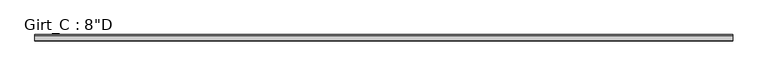
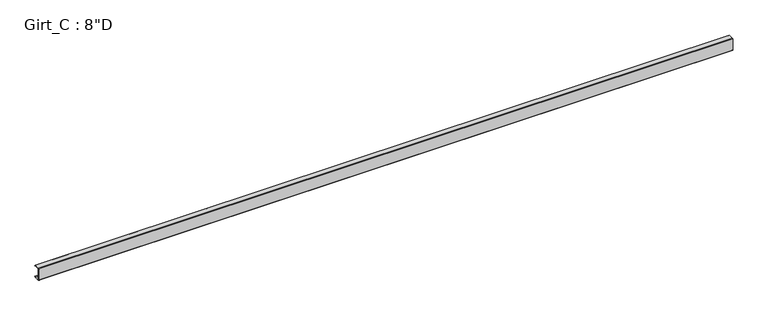
"""IFC4 building model written with IfcOpenShell, lengths in millimetres: beam geometry."""

import ifcopenshell
import ifcopenshell.guid

model = None  # the IFC model being written
_history = None  # IfcOwnerHistory: only IFC2X3 demands one
_inside = {}  # id of a spatial element -> (the spatial element, [elements in it])
_under = {}  # id of a project, library or spatial element -> (it, [spatial elements below it])
_declared = {}  # id of a project -> (the project, [libraries it declares])
_typed = {}  # id of a type object -> (the type object, [elements of that type])
_made_of = {}  # id of a material, layer set ... -> (it, [elements and type objects made of it])


def new_model(schema):
    """Start an empty IFC model of exactly this schema.

    Asked for "IFC4X3", IfcOpenShell would pick the latest addendum, in which some entities
    have other attributes; the version numbers below select the first issue.
    IFC2X3 requires an IfcOwnerHistory on every rooted entity: one is made here for all.
    """
    global model, _history
    if schema == "IFC4X3":
        model = ifcopenshell.file(schema_version=(4, 3, 0, 0))
    else:
        model = ifcopenshell.file(schema=schema)
    _inside.clear()
    _under.clear()
    _declared.clear()
    _typed.clear()
    _made_of.clear()
    _history = None
    if model.schema == "IFC2X3":
        org = make("IfcOrganization", Name="unknown")
        user = make(
            "IfcPersonAndOrganization",
            ThePerson=make("IfcPerson", FamilyName="unknown"),
            TheOrganization=org,
        )
        app = make(
            "IfcApplication",
            ApplicationDeveloper=org,
            Version="unknown",
            ApplicationFullName="unknown",
            ApplicationIdentifier="unknown",
        )
        _history = make(
            "IfcOwnerHistory",
            OwningUser=user,
            OwningApplication=app,
            ChangeAction="ADDED",
            CreationDate=0,
        )
    return model


def make(cls, **values):
    """One entity of the class cls with the attributes given. An attribute that is None is left unset."""
    return model.create_entity(
        cls, **{name: value for name, value in values.items() if value is not None}
    )


def rooted(cls, **values):
    """An entity with a GlobalId (a new one), such as an element, a storey or a relation."""
    return make(cls, GlobalId=ifcopenshell.guid.new(), OwnerHistory=_history, **values)


def si_unit(unit_type, name, prefix=None):
    """IfcSIUnit, for example si_unit("LENGTHUNIT", "METRE", prefix="MILLI")."""
    return make("IfcSIUnit", UnitType=unit_type, Prefix=prefix, Name=name)


def assignment(units):
    """IfcUnitAssignment: the units of a project."""
    return None if units is None else make("IfcUnitAssignment", Units=units)


def point(xyz):
    """IfcCartesianPoint."""
    return None if xyz is None else make("IfcCartesianPoint", Coordinates=xyz)


def direction(xyz):
    """IfcDirection."""
    return None if xyz is None else make("IfcDirection", DirectionRatios=xyz)


def frame(location, z_axis=None, x_axis=None):
    """IfcAxis2Placement3D, a coordinate frame: its origin and axes. An axis left out is left unset."""
    return make(
        "IfcAxis2Placement3D",
        Location=point(location),
        Axis=direction(z_axis),
        RefDirection=direction(x_axis),
    )


def frame_2d(location, x_axis=None):
    """IfcAxis2Placement2D, a coordinate frame in the plane: its origin and x axis."""
    return make(
        "IfcAxis2Placement2D", Location=point(location), RefDirection=direction(x_axis)
    )


def origin():
    """The frame at (0, 0, 0) with its axes left unset."""
    return frame((0.0, 0.0, 0.0))


def place(relative_to, where):
    """IfcLocalPlacement: puts the frame where relative to a parent placement (None: the world)."""
    return make(
        "IfcLocalPlacement", PlacementRelTo=relative_to, RelativePlacement=where
    )


def context(
    kind, dimensions, precision=None, world=None, true_north=None, identifier=None
):
    """IfcGeometricRepresentationContext, for example the 3D "Model" context."""
    return make(
        "IfcGeometricRepresentationContext",
        ContextIdentifier=identifier,
        ContextType=kind,
        CoordinateSpaceDimension=dimensions,
        Precision=precision,
        WorldCoordinateSystem=world,
        TrueNorth=true_north,
    )


def project(units=None, contexts=None):
    """IfcProject with its units and contexts."""
    return rooted(
        "IfcProject",
        Name="project",
        RepresentationContexts=contexts,
        UnitsInContext=assignment(units),
    )


def spatial(cls, under=None, at=None, **own):
    """A site, building, storey or space (cls), placed at a placement, below another one or the project."""
    s = rooted(cls, ObjectPlacement=at, **own)
    if under is not None:
        _under.setdefault(under.id(), (under, []))[1].append(s)
    return s


def polyline(points):
    """IfcPolyline through the points."""
    return make("IfcPolyline", Points=[point(p) for p in points])


def circle_curve(where, radius):
    """IfcCircle in the frame where."""
    return make("IfcCircle", Position=where, Radius=radius)


def trimmed(basis, trim1, trim2, sense, master):
    """IfcTrimmedCurve: the piece of a basis curve between two trims."""
    return make(
        "IfcTrimmedCurve",
        BasisCurve=basis,
        Trim1=trim1,
        Trim2=trim2,
        SenseAgreement=sense,
        MasterRepresentation=master,
    )


def segment(curve, same_sense, transition):
    """IfcCompositeCurveSegment."""
    return make(
        "IfcCompositeCurveSegment",
        Transition=transition,
        SameSense=same_sense,
        ParentCurve=curve,
    )


def composite_curve(segments, self_intersect=None):
    """IfcCompositeCurve: segments joined end to end."""
    return make("IfcCompositeCurve", Segments=segments, SelfIntersect=self_intersect)


def outline(outer, holes=None, kind="AREA"):
    """IfcArbitraryClosedProfileDef: a profile drawn as a closed curve; with holes, ...WithVoids."""
    if holes is None:
        return make("IfcArbitraryClosedProfileDef", ProfileType=kind, OuterCurve=outer)
    return make(
        "IfcArbitraryProfileDefWithVoids",
        ProfileType=kind,
        OuterCurve=outer,
        InnerCurves=holes,
    )


def extrude(swept, where, along, depth):
    """IfcExtrudedAreaSolid: the profile swept, set in the frame where, extruded along a direction by depth."""
    return make(
        "IfcExtrudedAreaSolid",
        SweptArea=swept,
        Position=where,
        ExtrudedDirection=direction(along),
        Depth=depth,
    )


def shape(context_of_items, identifier, shape_type, items):
    """IfcShapeRepresentation: the items that make up one representation, for example the "Body"."""
    return make(
        "IfcShapeRepresentation",
        ContextOfItems=context_of_items,
        RepresentationIdentifier=identifier,
        RepresentationType=shape_type,
        Items=items,
    )


def source(mapping_origin, context_of_items, identifier, shape_type, items):
    """IfcRepresentationMap: a shape defined once, which mapped items show again and again."""
    return make(
        "IfcRepresentationMap",
        MappingOrigin=mapping_origin,
        MappedRepresentation=shape(context_of_items, identifier, shape_type, items),
    )


def transform(
    local_origin,
    x_axis=None,
    y_axis=None,
    z_axis=None,
    scale=None,
    scale2=None,
    scale3=None,
    uniform=True,
):
    """IfcCartesianTransformationOperator3D, or its non-uniform kind. x_axis, y_axis, z_axis: its Axis1, 2, 3."""
    if uniform:
        return make(
            "IfcCartesianTransformationOperator3D",
            Axis1=direction(x_axis),
            Axis2=direction(y_axis),
            LocalOrigin=point(local_origin),
            Scale=scale,
            Axis3=direction(z_axis),
        )
    return make(
        "IfcCartesianTransformationOperator3DnonUniform",
        Axis1=direction(x_axis),
        Axis2=direction(y_axis),
        LocalOrigin=point(local_origin),
        Scale=scale,
        Axis3=direction(z_axis),
        Scale2=scale2,
        Scale3=scale3,
    )


def mapped(mapping_source, mapping_target):
    """IfcMappedItem: shows the shape of a source again, moved by a transform."""
    return make(
        "IfcMappedItem", MappingSource=mapping_source, MappingTarget=mapping_target
    )


def made_of(thing, what):
    """Note that an element or type object is made of a material, layer set ...; save() writes the relation."""
    if what is not None:
        _made_of.setdefault(what.id(), (what, []))[1].append(thing)
    return thing


def element(
    cls,
    number,
    at=None,
    inside=None,
    cuts=None,
    type_object=None,
    material=None,
    context=None,
    identifier="Body",
    shape_type=None,
    held_by="IfcProductDefinitionShape",
    body=None,
    shapes=None,
    **own,
):
    """One element of the class cls, such as IfcWall. Its Tag is "e" and its number.

    at: its placement. inside: the storey or other place that contains it. cuts: it is an
    opening in that element (IfcRelVoidsElement). A single representation is given by context,
    identifier, shape_type and body (its items); several are given by shapes. held_by: the class
    of the entity that holds the representations. save() writes the other relations.
    """
    e = rooted(cls, Tag="e%d" % number, ObjectPlacement=at, **own)
    if body is not None:
        shapes = [shape(context, identifier, shape_type, body)]
    if shapes is not None:
        e.Representation = make(held_by, Representations=shapes)
    if inside is not None:
        _inside.setdefault(inside.id(), (inside, []))[1].append(e)
    if cuts is not None:
        rooted(
            "IfcRelVoidsElement", RelatingBuildingElement=cuts, RelatedOpeningElement=e
        )
    if type_object is not None:
        _typed.setdefault(type_object.id(), (type_object, []))[1].append(e)
    return made_of(e, material)


def aggregate(whole, parts):
    """IfcRelAggregates: a whole, such as a stair, and the parts it consists of."""
    return rooted("IfcRelAggregates", RelatingObject=whole, RelatedObjects=parts)


def save(model, path):
    """Write the relations noted so far, then the file.

    IfcRelAggregates (storeys below a building ...), IfcRelContainedInSpatialStructure (elements
    in a storey), IfcRelDefinesByType, IfcRelAssociatesMaterial and IfcRelDeclares: one each for
    every whole, place, type object, material and project.
    """
    for whole, parts in _under.values():
        aggregate(whole, parts)
    for where, things in _inside.values():
        rooted(
            "IfcRelContainedInSpatialStructure",
            RelatedElements=things,
            RelatingStructure=where,
        )
    for kind, things in _typed.values():
        rooted("IfcRelDefinesByType", RelatedObjects=things, RelatingType=kind)
    for what, things in _made_of.values():
        rooted("IfcRelAssociatesMaterial", RelatedObjects=things, RelatingMaterial=what)
    for by, libraries in _declared.values():
        rooted("IfcRelDeclares", RelatingContext=by, RelatedDefinitions=libraries)
    model.write(path)


def beam_95505e83(model_context):
    return source(origin(), model_context, "Body", "SweptSolid", [
        extrude(outline(composite_curve([segment(polyline([(87.5109375, 101.6), (99.7560415, 87.0068534), (97.6278742, 85.221109), (86.2154765, 98.821875), (3.3005807, 98.821875)]), True, "CONTINUOUS"), segment(trimmed(circle_curve(frame_2d((3.3741066, 96.8381931)), 1.9850441), [point((3.3005807, 98.821875))], [point((1.3890625, 96.8381931))], True, "CARTESIAN"), True, "CONTINUOUS"), segment(polyline([(1.3890625, 96.8381931), (1.3890625, -96.8389339)]), True, "CONTINUOUS"), segment(trimmed(circle_curve(frame_2d((3.3748024, -96.8389339)), 1.9857399), [point((1.3890625, -96.8389339))], [point((3.2694106, -98.821875))], True, "CARTESIAN"), True, "CONTINUOUS"), segment(polyline([(3.2694106, -98.821875), (86.2154765, -98.821875), (97.6510975, -85.1934327), (99.7792647, -86.979177), (87.5109375, -101.6), (3.3734375, -101.6)]), True, "CONTINUOUS"), segment(trimmed(circle_curve(frame_2d((3.3734375, -96.8375)), 4.7625), [point((3.3734375, -101.6))], [point((-1.3890625, -96.8375))], False, "CARTESIAN"), True, "CONTINUOUS"), segment(polyline([(-1.3890625, -96.8375), (-1.3890625, 96.8375)]), True, "CONTINUOUS"), segment(trimmed(circle_curve(frame_2d((3.3734375, 96.8375)), 4.7625), [point((-1.3890625, 96.8375))], [point((3.3734375, 101.6))], False, "CARTESIAN"), True, "CONTINUOUS"), segment(polyline([(3.3734375, 101.6), (87.5109375, 101.6)]), True, "CONTINUOUS")], self_intersect=False)), frame((-5621.3960998, 0.0, 0.0), z_axis=(1.0, 0.0, 0.0), x_axis=(0.0, 1.0, 0.0)), (0.0, 0.0, 1.0), 11076.8984495),
    ])


if __name__ == "__main__":
    model = new_model("IFC4")
    model_context = context("Model", 3, world=origin())
    ifc_project = project(units=[si_unit("LENGTHUNIT", "METRE", prefix="MILLI")], contexts=[model_context])
    site = spatial("IfcSite", under=ifc_project)
    building = spatial("IfcBuilding", under=site)
    placement = place(None, origin())
    beam_shape = beam_95505e83(model_context)
    element("IfcBeam", 1, ObjectType="Girt_C : 8\"D", at=placement, inside=building, context=model_context, shape_type="MappedRepresentation", body=[
        mapped(beam_shape, transform((0.0, 0.0, 0.0), x_axis=(1.0, 0.0, 0.0), y_axis=(0.0, 1.0, 0.0), z_axis=(0.0, 0.0, 1.0))),
    ])
    save(model, "model.ifc")

# Revit data of these elements
# Type "Girt_C : 8\"D"
#   half leg = 0' - 1 3/4"
#   Web_Thickness = 0' - 0 7/64"
#   Length [instance default] = 10' - 0"
#   Leg_1 = 0' - 3 1/2"
#   Height = 0' - 8"
#   Structural Material [instance default] = none
# Element 1 (IfcBeam, "Girt_C : 8\"D")
#   Structural Material = GALVANIZED 'CEE' SECTION (8.0x3.5C - SEE STRUCT. DWGS)
#   Materials on its faces: "GALVANIZED 'CEE' SECTION (8.0x3.5C - SEE STRUCT. DWGS)"
# Materials
#   "GALVANIZED 'CEE' SECTION (8.0x3.5C - SEE STRUCT. DWGS)": class "Metal", colour RGB 137 146 153, transparency 0, Description = "Steel, mill finish", Cost = 0
